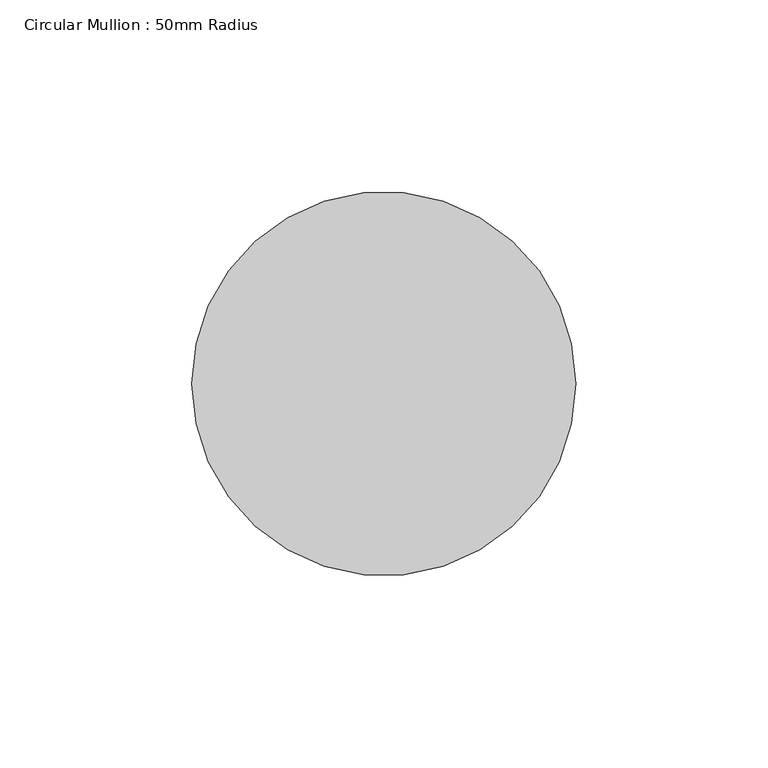
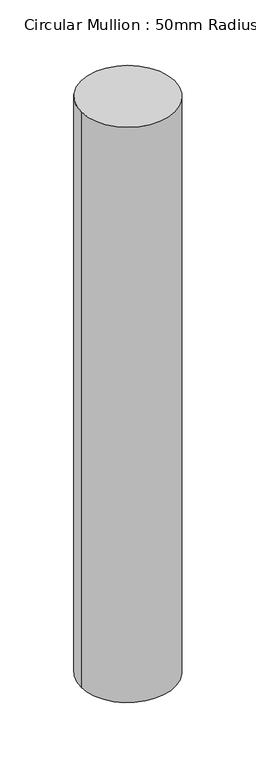
"""IFC4 building model written with IfcOpenShell, lengths in millimetres: member geometry, Circular Mullion : 50mm Radius."""

from ifc_helpers import new_model, si_unit, point, frame, origin, origin_2d, place, context, project, spatial, circle_curve, trimmed, segment, composite_curve, outline, extrude, source, transform, mapped, element, save


def circular_mullion_50mm_radius_67650c96(model_context):
    return source(origin(), model_context, "Body", "SweptSolid", [
        extrude(outline(composite_curve([segment(trimmed(circle_curve(origin_2d(), 50.0), [point((50.0, 0.0))], [point((-50.0, 0.0))], False, "CARTESIAN"), True, "CONTINUOUS"), segment(trimmed(circle_curve(origin_2d(), 50.0), [point((-50.0, 0.0))], [point((50.0, 0.0))], False, "CARTESIAN"), True, "CONTINUOUS")], self_intersect=False)), frame((0.0, 0.0, -649.9247327), z_axis=(0.0, 0.0, 1.0), x_axis=(1.0, 0.0, 0.0)), (0.0, 0.0, 1.0), 649.9247327),
    ])


if __name__ == "__main__":
    model = new_model("IFC4")
    model_context = context("Model", 3, world=origin())
    ifc_project = project(units=[si_unit("LENGTHUNIT", "METRE", prefix="MILLI")], contexts=[model_context])
    site = spatial("IfcSite", under=ifc_project)
    building = spatial("IfcBuilding", under=site)
    placement = place(None, origin())
    circular_mullion_50mm_radius_shape = circular_mullion_50mm_radius_67650c96(model_context)
    element("IfcMember", 1, ObjectType="Circular Mullion : 50mm Radius", at=placement, inside=building, context=model_context, shape_type="MappedRepresentation", body=[
        mapped(circular_mullion_50mm_radius_shape, transform((0.0, 0.0, 0.0), x_axis=(1.0, 0.0, 0.0), y_axis=(0.0, 1.0, 0.0), z_axis=(0.0, 0.0, 1.0))),
    ])
    save(model, "model.ifc")

# Revit data of these elements
# Type "Circular Mullion : 50mm Radius"
#   built-in parameter 1007350 = 0.164042 (stored number, unit not read)
# Element 1 (IfcMember, "Circular Mullion : 50mm Radius")
#   Materials on its faces: "Aluminium"
# Materials
#   "Aluminium": class "Metal", colour RGB 247 247 247, transparency 0, Description = "Aluminium 6061", Cost = 0
